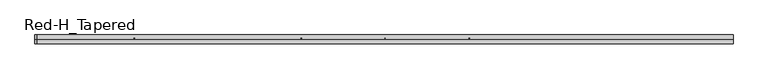
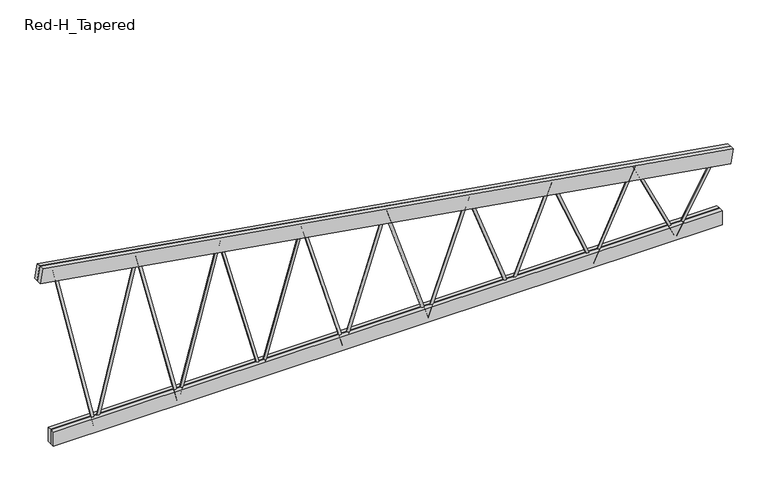
"""IFC4 building model written with IfcOpenShell, lengths in millimetres: beam geometry, Construction_Frames_RedBuilt_Openweb_Red-H_Tapered : Red-H_Tapered."""

from ifc_helpers import new_model, si_unit, point, frame, origin, origin_2d, place, context, project, spatial, polyline, circle_curve, trimmed, segment, composite_curve, outline, extrude, source, transform, mapped, element, save


def red_h_tapered_c7778fd0(model_context):
    return source(origin(), model_context, "Body", "SweptSolid", [
        extrude(outline(composite_curve([segment(trimmed(circle_curve(origin_2d(), 12.7), [point((0.0, -12.7))], [point((0.0, 12.7000001))], False, "CARTESIAN"), True, "CONTINUOUS"), segment(trimmed(circle_curve(origin_2d(), 12.7), [point((0.0, 12.7000001))], [point((0.0, -12.7))], False, "CARTESIAN"), True, "CONTINUOUS")], self_intersect=False)), frame((-384.3734375, 0.0, -417.8101562), z_axis=(-0.2818839214025414, 0.0, 0.9594485160000645), x_axis=(0.0, 1.0, 0.0)), (0.0, 0.0, 1.0), 1363.5876626),
        extrude(outline(composite_curve([segment(trimmed(circle_curve(origin_2d(), 12.7), [point((0.0, 12.7))], [point((0.0, -12.7000001))], False, "CARTESIAN"), True, "CONTINUOUS"), segment(trimmed(circle_curve(origin_2d(), 12.7), [point((0.0, -12.7000001))], [point((0.0, 12.7))], False, "CARTESIAN"), True, "CONTINUOUS")], self_intersect=False)), frame((-1153.1203125, 0.0, -417.8101562), z_axis=(0.2818839214025404, 0.0, 0.9594485160000648), x_axis=(0.0, 1.0, 0.0)), (0.0, 0.0, 1.0), 1363.5876626),
        extrude(outline(composite_curve([segment(trimmed(circle_curve(origin_2d(), 12.7), [point((0.0, -12.6999999))], [point((0.0, 12.7))], False, "CARTESIAN"), True, "CONTINUOUS"), segment(trimmed(circle_curve(origin_2d(), 12.7), [point((0.0, 12.7))], [point((0.0, -12.6999999))], False, "CARTESIAN"), True, "CONTINUOUS")], self_intersect=False)), frame((-1153.1203125, 0.0, -417.8101562), z_axis=(-0.2591073148814879, 0.0, 0.9658485385270847), x_axis=(0.0, 1.0, 0.0)), (0.0, 0.0, 1.0), 1483.4526678),
        extrude(outline(composite_curve([segment(trimmed(circle_curve(origin_2d(), 12.7), [point((0.0, 12.6999999))], [point((0.0, -12.7))], False, "CARTESIAN"), True, "CONTINUOUS"), segment(trimmed(circle_curve(origin_2d(), 12.7), [point((0.0, -12.7))], [point((0.0, 12.6999999))], False, "CARTESIAN"), True, "CONTINUOUS")], self_intersect=False)), frame((-1921.8671875, 0.0, -417.8101562), z_axis=(0.2591073148814962, 0.0, 0.9658485385270825), x_axis=(0.0, 1.0, 0.0)), (0.0, 0.0, 1.0), 1483.4526678),
        extrude(outline(composite_curve([segment(trimmed(circle_curve(origin_2d(), 12.7), [point((0.0, -12.7))], [point((0.0, 12.7))], False, "CARTESIAN"), True, "CONTINUOUS"), segment(trimmed(circle_curve(origin_2d(), 12.7), [point((0.0, 12.7))], [point((0.0, -12.7))], False, "CARTESIAN"), True, "CONTINUOUS")], self_intersect=False)), frame((-1921.8671875, 0.0, -417.8101562), z_axis=(-0.23963077149041714, 0.0, 0.9708640962333027), x_axis=(0.0, 1.0, 0.0)), (0.0, 0.0, 1.0), 1604.0237033),
        extrude(outline(composite_curve([segment(trimmed(circle_curve(origin_2d(), 12.7), [point((0.0, 12.7))], [point((0.0, -12.7))], False, "CARTESIAN"), True, "CONTINUOUS"), segment(trimmed(circle_curve(origin_2d(), 12.7), [point((0.0, -12.7))], [point((0.0, 12.7))], False, "CARTESIAN"), True, "CONTINUOUS")], self_intersect=False)), frame((-2690.6140625, 0.0, -417.8101562), z_axis=(0.23963077149041034, 0.0, 0.9708640962333044), x_axis=(0.0, 1.0, 0.0)), (0.0, 0.0, 1.0), 1604.0237033),
        extrude(outline(composite_curve([segment(trimmed(circle_curve(origin_2d(), 12.7), [point((0.0, -12.7))], [point((0.0, 12.7))], False, "CARTESIAN"), True, "CONTINUOUS"), segment(trimmed(circle_curve(origin_2d(), 12.7), [point((0.0, 12.7))], [point((0.0, -12.7))], False, "CARTESIAN"), True, "CONTINUOUS")], self_intersect=False)), frame((-2690.6140625, 0.0, -417.8101562), z_axis=(-0.22280545262596763, 0.0, 0.9748629289700874), x_axis=(0.0, 1.0, 0.0)), (0.0, 0.0, 1.0), 1725.1527419),
        extrude(outline(composite_curve([segment(trimmed(circle_curve(origin_2d(), 12.7), [point((0.0, -12.7000001))], [point((0.0, 12.7))], False, "CARTESIAN"), True, "CONTINUOUS"), segment(trimmed(circle_curve(origin_2d(), 12.7), [point((0.0, 12.7))], [point((0.0, -12.7000001))], False, "CARTESIAN"), True, "CONTINUOUS")], self_intersect=False)), frame((2690.6140625, 0.0, -417.8101562), z_axis=(0.48891846545083756, 0.0, 0.8723294871441629), x_axis=(0.0, 1.0, 0.0)), (0.0, 0.0, 1.0), 786.1708335),
        extrude(outline(composite_curve([segment(trimmed(circle_curve(origin_2d(), 12.7), [point((0.0, 12.7))], [point((0.0, -12.6999999))], False, "CARTESIAN"), True, "CONTINUOUS"), segment(trimmed(circle_curve(origin_2d(), 12.7), [point((0.0, -12.6999999))], [point((0.0, 12.7))], False, "CARTESIAN"), True, "CONTINUOUS")], self_intersect=False)), frame((2690.6140625, 0.0, -417.8101562), z_axis=(-0.4285852121446376, 0.0, 0.9035013646536103), x_axis=(0.0, 1.0, 0.0)), (0.0, 0.0, 1.0), 896.8425102),
        extrude(outline(composite_curve([segment(trimmed(circle_curve(origin_2d(), 12.7), [point((0.0, -12.7))], [point((0.0, 12.6999999))], False, "CARTESIAN"), True, "CONTINUOUS"), segment(trimmed(circle_curve(origin_2d(), 12.7), [point((0.0, 12.6999999))], [point((0.0, -12.7))], False, "CARTESIAN"), True, "CONTINUOUS")], self_intersect=False)), frame((1921.8671875, 0.0, -417.8101562), z_axis=(0.42858521214463685, 0.0, 0.9035013646536108), x_axis=(0.0, 1.0, 0.0)), (0.0, 0.0, 1.0), 896.8425102),
        extrude(outline(composite_curve([segment(trimmed(circle_curve(origin_2d(), 12.7), [point((0.0, 12.7))], [point((0.0, -12.7))], False, "CARTESIAN"), True, "CONTINUOUS"), segment(trimmed(circle_curve(origin_2d(), 12.7), [point((0.0, -12.7))], [point((0.0, 12.7))], False, "CARTESIAN"), True, "CONTINUOUS")], self_intersect=False)), frame((1921.8671875, 0.0, -417.8101562), z_axis=(-0.3802904782348009, 0.0, 0.9248670997305215), x_axis=(0.0, 1.0, 0.0)), (0.0, 0.0, 1.0), 1010.7364225),
        extrude(outline(composite_curve([segment(trimmed(circle_curve(origin_2d(), 12.7), [point((0.0, -12.7))], [point((0.0, 12.7))], False, "CARTESIAN"), True, "CONTINUOUS"), segment(trimmed(circle_curve(origin_2d(), 12.7), [point((0.0, 12.7))], [point((0.0, -12.7))], False, "CARTESIAN"), True, "CONTINUOUS")], self_intersect=False)), frame((1153.1203125, 0.0, -417.8101562), z_axis=(0.38029047823480006, 0.0, 0.924867099730522), x_axis=(0.0, 1.0, 0.0)), (0.0, 0.0, 1.0), 1010.7364225),
        extrude(outline(composite_curve([segment(trimmed(circle_curve(origin_2d(), 12.7), [point((0.0, 12.7))], [point((0.0, -12.7))], False, "CARTESIAN"), True, "CONTINUOUS"), segment(trimmed(circle_curve(origin_2d(), 12.7), [point((0.0, -12.7))], [point((0.0, 12.7))], False, "CARTESIAN"), True, "CONTINUOUS")], self_intersect=False)), frame((1153.1203125, 0.0, -417.8101562), z_axis=(-0.3410964880623186, 0.0, 0.9400282899102306), x_axis=(0.0, 1.0, 0.0)), (0.0, 0.0, 1.0), 1126.8759748),
        extrude(outline(composite_curve([segment(trimmed(circle_curve(origin_2d(), 12.7), [point((0.0, -12.7))], [point((0.0, 12.7))], False, "CARTESIAN"), True, "CONTINUOUS"), segment(trimmed(circle_curve(origin_2d(), 12.7), [point((0.0, 12.7))], [point((0.0, -12.7))], False, "CARTESIAN"), True, "CONTINUOUS")], self_intersect=False)), frame((384.3734375, 0.0, -417.8101562), z_axis=(0.34109648806231907, 0.0, 0.9400282899102305), x_axis=(0.0, 1.0, 0.0)), (0.0, 0.0, 1.0), 1126.8759748),
        extrude(outline(composite_curve([segment(trimmed(circle_curve(origin_2d(), 12.7), [point((0.0, 12.7))], [point((0.0, -12.7))], False, "CARTESIAN"), True, "CONTINUOUS"), segment(trimmed(circle_curve(origin_2d(), 12.7), [point((0.0, -12.7))], [point((0.0, 12.7))], False, "CARTESIAN"), True, "CONTINUOUS")], self_intersect=False)), frame((384.3734375, 0.0, -417.8101562), z_axis=(-0.3088247971808634, 0.0, 0.9511189434798356), x_axis=(0.0, 1.0, 0.0)), (0.0, 0.0, 1.0), 1244.6326882),
        extrude(outline(composite_curve([segment(trimmed(circle_curve(origin_2d(), 12.7), [point((0.0, 12.7))], [point((0.0, -12.7))], False, "CARTESIAN"), True, "CONTINUOUS"), segment(trimmed(circle_curve(origin_2d(), 12.7), [point((0.0, -12.7))], [point((0.0, 12.7))], False, "CARTESIAN"), True, "CONTINUOUS")], self_intersect=False)), frame((-384.3734375, 0.0, -417.8101562), z_axis=(0.3088247971808418, 0.0, 0.9511189434798426), x_axis=(0.0, 1.0, 0.0)), (0.0, 0.0, 1.0), 1244.6326882),
        extrude(outline(polyline([(-3100.3875, 41.275), (3100.3875, 41.275), (3100.3875, 3.175), (-3100.3875, 3.175), (-3100.3875, 41.275)])), frame((0.0, 0.0, -436.8601562), z_axis=(0.0, 0.0, 1.0), x_axis=(1.0, 0.0, 0.0)), (0.0, 0.0, 1.0), 139.7),
        extrude(outline(polyline([(-3100.3875, -3.175), (3100.3875, -3.175), (3100.3875, -41.275), (-3100.3875, -41.275), (-3100.3875, -3.175)])), frame((0.0, 0.0, -436.8601562), z_axis=(0.0, 0.0, 1.0), x_axis=(1.0, 0.0, 0.0)), (0.0, 0.0, 1.0), 139.7),
        extrude(outline(polyline([(0.0, 38.1), (6492.222889, 38.1), (6492.222889, 0.0), (0.0, 0.0), (0.0, 38.1)])), frame((-3224.9429596, 3.175, 1203.3387666), z_axis=(0.16431968190823515, 0.0, 0.986407138121768), x_axis=(0.986407138121768, 0.0, -0.16431968190823515)), (0.0, 0.0, 1.0), 139.7),
        extrude(outline(polyline([(0.0, 38.1), (6492.222889, 38.1), (6492.222889, 0.0), (0.0, 0.0), (0.0, 38.1)])), frame((-3224.9429596, -41.275, 1203.3387666), z_axis=(0.16431968190823515, 0.0, 0.986407138121768), x_axis=(0.986407138121768, 0.0, -0.16431968190823515)), (0.0, 0.0, 1.0), 139.7),
    ])


if __name__ == "__main__":
    model = new_model("IFC4")
    model_context = context("Model", 3, world=origin())
    ifc_project = project(units=[si_unit("LENGTHUNIT", "METRE", prefix="MILLI")], contexts=[model_context])
    site = spatial("IfcSite", under=ifc_project)
    building = spatial("IfcBuilding", under=site)
    placement = place(None, origin())
    red_h_tapered_shape = red_h_tapered_c7778fd0(model_context)
    element("IfcBeam", 1, ObjectType="Construction_Frames_RedBuilt_Openweb_Red-H_Tapered : Red-H_Tapered", at=placement, inside=building, context=model_context, shape_type="MappedRepresentation", body=[
        mapped(red_h_tapered_shape, transform((0.0, 0.0, 0.0), x_axis=(1.0, 0.0, 0.0), y_axis=(0.0, 1.0, 0.0), z_axis=(0.0, 0.0, 1.0))),
    ])
    save(model, "model.ifc")

# Revit data of these elements
# Type "Construction_Frames_RedBuilt_Openweb_Red-H_Tapered : Red-H_Tapered"
#   Youtube clip = ""
#   Weight Net (Kg) = "0"
#   Webs = "Up to 2\" diameter tubular steel"
#   Uniformat II Description = ""
#   Uniformat II Code = ""
#   Uniclass 2015 Name = "Softwood trusses"
#   Uniclass 2015 Code = "Pr_20_85_90_81"
#   Uniclass 2.0 Description = "Structural Framing Systems"
#   Uniclass 2.0 Code = "SS-15-10-75"
#   Uniclass 1.4 Description = "Trusses"
#   Uniclass 1.4 Code = "L3523"
#   UNSPSC Code = "30103606"
#   Technical description = "http://www.redbuilt.com/reference/literature-and-other-resources"
#   Region South America = "None"
#   Region Oceania = "None"
#   Region North America = "US"
#   Region Middle East = "None"
#   Region Europe = "None"
#   Region Asia = "None"
#   Region Antarctica = "None"
#   Region Africa = "None"
#   QR code = "http://bimobject.com/redbuilt/product/redbuilt-0003"
#   Product url = "http://www.redbuilt.com/products/default.aspx?id=2"
#   Product group = "Wood Trusses"
#   Product family = "Construction"
#   Product data url = "https://bimobject.com/redbuilt/product/redbuilt-0003"
#   Product certification = ""
#   Product SKU = "redbuilt-0003"
#   Product Page URL = "http://www.redbuilt.com/commercial-systems/red-m-red-h-open-web-trusses"
#   Product Guid = "2c5793f2-6ffb-4665-b825-cf90c048e711"
#   Product Documentation Link = "http://www.redbuilt.com/documents/OW_Guide_2017_07_LowRes_wLinks.pdf"
#   OmniClass Description = "Wood Trusses"
#   OmniClass Code = "23-13 35 19 13 17"
#   NBS Reference Description = ""
#   NBS Reference Code = ""
#   Material secondary = "Steel"
#   Material main = "CHARRED WOOD"
#   Masterformat 2014 Description = "Metal-Web Wood Joists"
#   Masterformat 2014 Code = "06 17 36"
#   Manufacturer name = "RedBuilt"
#   Manufacturer country = "United States"
#   Installation instructions = "http://www.redbuilt.com/documents/Installation_Sheets_Open-Web.pdf"
#   IFC Classification = ""
#   EAN code = ""
#   Design country = "United States"
#   Product Information = "http://redbuilt.com/products/default.aspx?id=2"
#   Model = "Red-H-Tapered"
#   Manufacturer URL = "http://redbuilt.com/"
#   Manufacturer = "RedBuilt™"
#   Description = "Open Web Truss"
#   Date of publishing = "8/17/2010"
#   Contact us = "http://redbuilt.com/contact/"
#   Chords = "Double 1½\" x 5½\" MSR lumber"
#   COBIe Type Category = ""
#   Brand url = "http://www.redbuilt.com"
#   BIMobject main category code = "construction"
#   BIMobject main category = "Construction"
#   BIMobject category code = "construction-frames-trusses"
#   BIMobject category = "Frames & Trusses"
#   Web Radius = 0' - 0 1/2"
#   Web Layout Offset Start [instance default] = 0' - 5"
#   Web Layout Offset End [instance default] = 0' - 5"
#   Web Diameter = 0' - 1"
#   TotalLength [instance default] = 20' - 0"
#   Span Minimum = 4' - 0"
#   Span Maximum = 70' - 0"
#   Span Limit [instance default] = 20' - 0"
#   Nominal width = 0' - 0"
#   Nominal height = 0' - 0"
#   Inner Depth Top [instance default] = 0' - 2.76372"
#   Depth Start [instance default] = 6' - 0"
#   Top Chord Length [instance default] = 20' - 1.19701"
#   TC Extension Start Aux [instance default] = 0' - 0"
#   TC Extension End Aux [instance default] = 0' - 0"
#   T-B Chord Length Difference L [instance default] = 0' - 4"
#   T-B Chord Length Difference [instance default] = 0' - 4"
#   Height 2 [instance default] = 6' - 0"
#   Depth Minimum at Wall = 2' - 0"
#   Depth Maximum at Wall = 6' - 0"
#   Depth Lower End [instance default] = 2' - 0"
#   Depth Higher End [instance default] = 6' - 0"
#   Depth End [instance default] = 2' - 0"
#   Depth 2 [instance default] = 2' - 0"
#   Chord Width = 0' - 3 1/4"
#   Chord Thickness = 0' - 1 1/2"
#   Chord Depth = 0' - 5 1/2"
#   Offset Start [instance default] = 0' - 0"
#   TC Extension Start [instance default] = 0' - 0"
#   End Panel = 0' - 5"
#   Offset End [instance default] = 0' - 0"
#   TC Extension End [instance default] = 0' - 0"
#   Length [instance default] = 20' - 0"
#   Angle [instance default] = 5.71059°
#   Span Limit Warning [instance default] = no
#   Edition number = 1
#   Top Bearing Start [instance default] = yes
#   Top Bearing End [instance default] = yes
#   Bottom Bearing Start [instance default] = no
#   Bottom Bearing End [instance default] = no
#   8 Panels [instance default] = yes
#   16 Panels [instance default] = no
#   12 Panels [instance default] = no
#   Web Material = RedBuilt-Steel, Galvanized
#   Clip Material = RedBuilt-Steel, Galvanized
#   Chords Material = WOOD-OAKFIRE
#   URL = ""
#   Assembly Code = ""
# Element 1 (IfcBeam, "Construction_Frames_RedBuilt_Openweb_Red-H_Tapered : Red-H_Tapered")
#   TotalLength = 21' - 0 1/8"
#   Span Limit = 21' - 0 1/8"
#   Inner Depth Top = 0' - 2.7879"
#   Depth Start = 5' - 0"
#   Top Chord Length = 21' - 3.59933"
#   Height 2 = 5' - 0"
#   Depth Lower End = 2' - 4"
#   Depth Higher End = 5' - 0"
#   Depth End = 2' - 4"
#   Depth 2 = 3' - 6"
#   Angle = 9.45772°
#   Materials on its faces: "RedBuilt-Steel, Galvanized", "WOOD-OAKFIRE"
# Materials
#   "RedBuilt-Steel, Galvanized": class "Metal", colour RGB 164 172 176, transparency 0, Manufacturer = "RedBuilt. LLC", Comments = "Openweb Metal Web", URL = "http://www.redbuilt.com/", Description = "Galvanized steel", Cost = 0
#   "WOOD-OAKFIRE": class "Wood", colour RGB 198 202 183, transparency 0, Description = "Generic wood", Cost = 0
